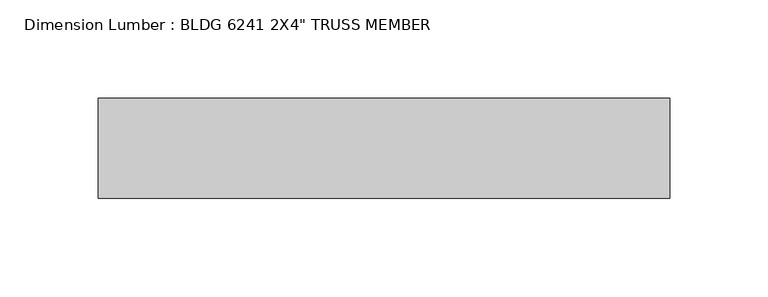
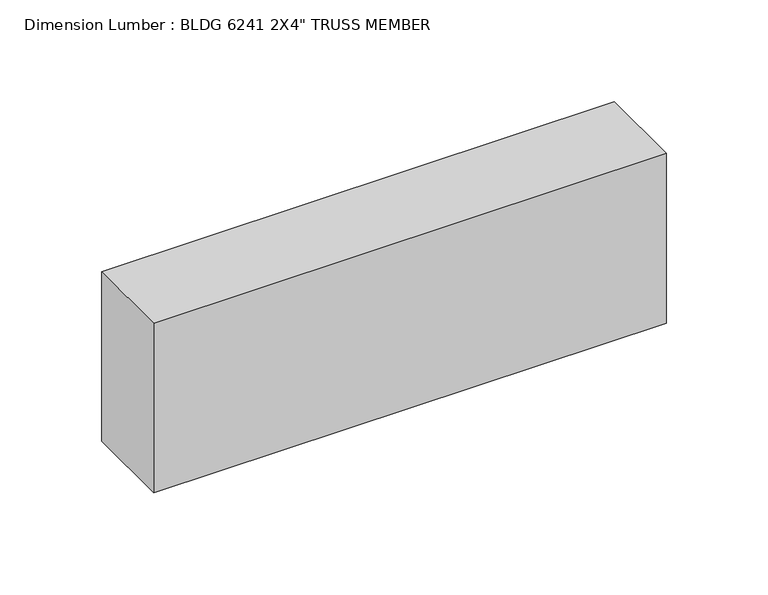
"""IFC4 building model written with IfcOpenShell, lengths in millimetres: beam geometry."""

from ifc_helpers import new_model, si_unit, frame, origin, place, context, project, spatial, polyline, outline, extrude, source, transform, mapped, element, save


def beam_11c5b8ca(model_context):
    return source(origin(), model_context, "Body", "SweptSolid", [
        extrude(outline(polyline([(147.1272806, -25.4), (-142.875, -25.4), (-142.875, 25.4), (147.1272806, 25.4), (147.1272806, -25.4)])), frame((0.0, 0.0, -50.8), z_axis=(0.0, 0.0, 1.0), x_axis=(1.0, 0.0, 0.0)), (0.0, 0.0, 1.0), 101.6),
    ])


if __name__ == "__main__":
    model = new_model("IFC4")
    model_context = context("Model", 3, world=origin())
    ifc_project = project(units=[si_unit("LENGTHUNIT", "METRE", prefix="MILLI")], contexts=[model_context])
    site = spatial("IfcSite", under=ifc_project)
    building = spatial("IfcBuilding", under=site)
    placement = place(None, origin())
    beam_shape = beam_11c5b8ca(model_context)
    element("IfcBeam", 1, ObjectType="Dimension Lumber : BLDG 6241 2X4\" TRUSS MEMBER", at=placement, inside=building, context=model_context, shape_type="MappedRepresentation", body=[
        mapped(beam_shape, transform((0.0, 0.0, 0.0), x_axis=(1.0, 0.0, 0.0), y_axis=(0.0, 1.0, 0.0), z_axis=(0.0, 0.0, 1.0))),
    ])
    save(model, "model.ifc")

# Revit data of these elements
# Type "Dimension Lumber : BLDG 6241 2X4\" TRUSS MEMBER"
#   Assembly Code = "B10"
#   A = 0.273472 SF
#   Length [instance default] = 5' - 0"
#   b = 0' - 2"
#   d = 0' - 4"
#   Structural Material [instance default] = Softwood, Lumber
# Element 1 (IfcBeam, "Dimension Lumber : BLDG 6241 2X4\" TRUSS MEMBER")
#   Materials on its faces: "Softwood, Lumber"
# Materials
#   "Softwood, Lumber": class "Wood", colour RGB 223 192 134, transparency 0, Description = "Pinus Echinata", Cost = 0
